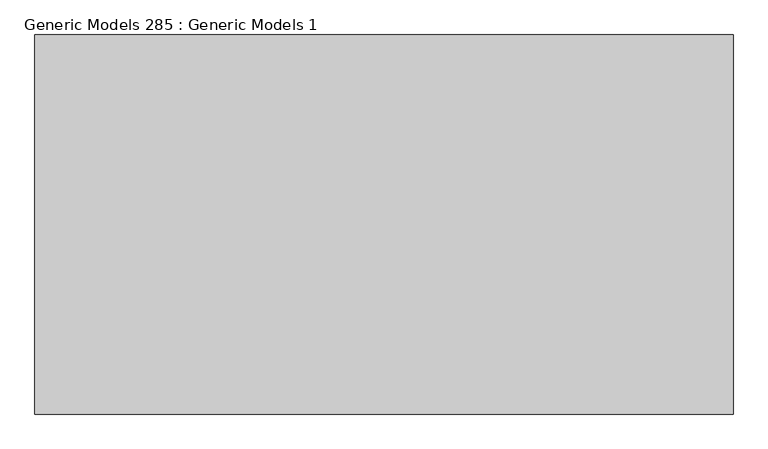
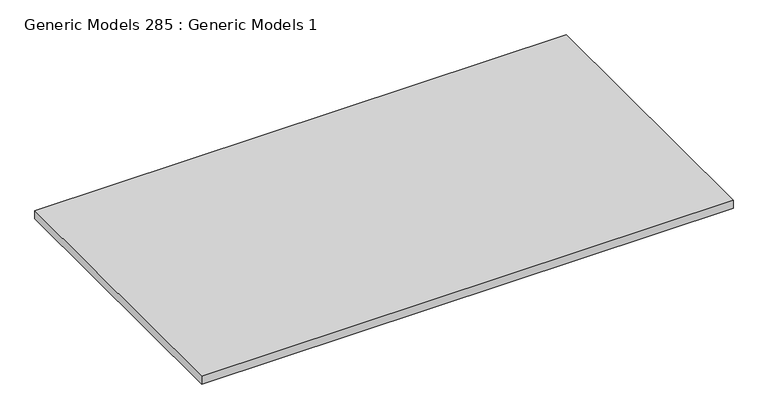
"""IFC4 building model written with IfcOpenShell, lengths in millimetres: proxy geometry, Generic Models 285 : Generic Models 1."""

from ifc_helpers import new_model, si_unit, frame, origin, place, context, project, spatial, polyline, outline, extrude, source, transform, mapped, element, save


def generic_models_285_generic_models_1_e29290d5(model_context):
    return source(origin(), model_context, "Body", "SweptSolid", [
        extrude(outline(polyline([(3397.147104, 1085.2769662), (4659.5673205, 1085.2769662), (4659.5673205, 399.7309662), (3397.147104, 399.7309662), (3397.147104, 1085.2769662)])), frame((0.0, 0.0, 126783.846), z_axis=(0.0, 0.0, 1.0), x_axis=(1.0, 0.0, 0.0)), (0.0, 0.0, 1.0), 19.05),
    ])


if __name__ == "__main__":
    model = new_model("IFC4")
    model_context = context("Model", 3, world=origin())
    ifc_project = project(units=[si_unit("LENGTHUNIT", "METRE", prefix="MILLI")], contexts=[model_context])
    site = spatial("IfcSite", under=ifc_project)
    building = spatial("IfcBuilding", under=site)
    placement = place(None, origin())
    generic_models_285_generic_models_1_shape = generic_models_285_generic_models_1_e29290d5(model_context)
    element("IfcBuildingElementProxy", 1, Name="Generic Models 285 : Generic Models 1", ObjectType="Generic Models 285 : Generic Models 1", at=placement, inside=building, context=model_context, shape_type="MappedRepresentation", body=[
        mapped(generic_models_285_generic_models_1_shape, transform((0.0, 0.0, 0.0), x_axis=(1.0, 0.0, 0.0), y_axis=(0.0, 1.0, 0.0), z_axis=(0.0, 0.0, 1.0))),
    ])
    save(model, "model.ifc")

# Revit data of these elements
# Element 1 (IfcBuildingElementProxy, "Generic Models 285 : Generic Models 1")
#   Materials on its faces: "_CDX PLYWOOD - SEE STRUCT DWGs"
# Materials
#   "_CDX PLYWOOD - SEE STRUCT DWGs": class "Generic", colour RGB 98 75 74, transparency 0, Cost = 0
